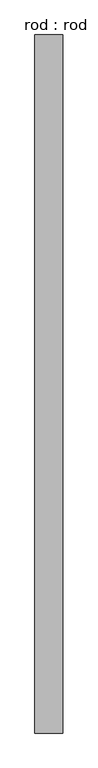
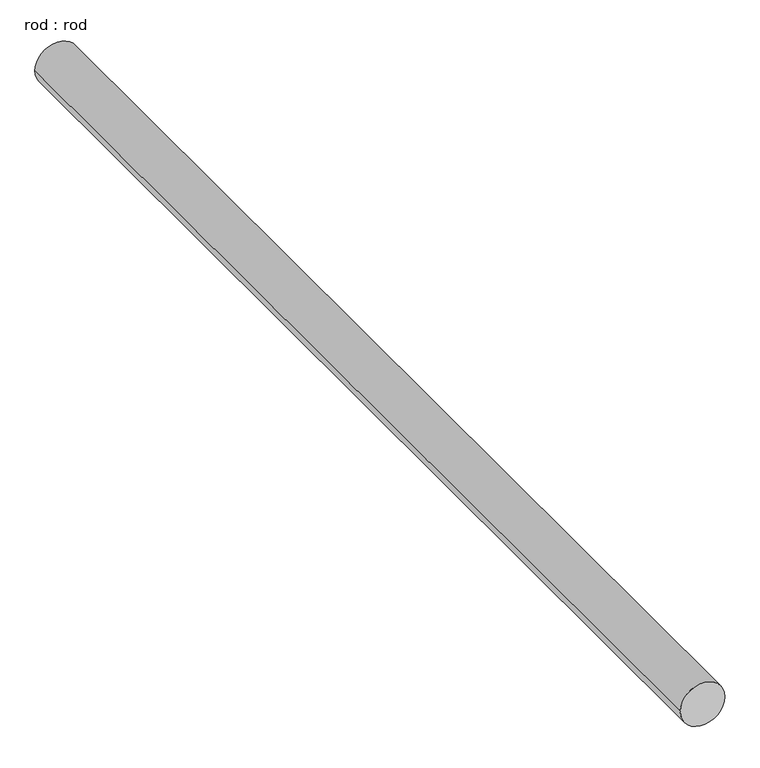
"""IFC4 building model written with IfcOpenShell, lengths in millimetres: proxy geometry, rod : rod."""

import ifcopenshell
import ifcopenshell.guid

model = None  # the IFC model being written
_history = None  # IfcOwnerHistory: only IFC2X3 demands one
_inside = {}  # id of a spatial element -> (the spatial element, [elements in it])
_under = {}  # id of a project, library or spatial element -> (it, [spatial elements below it])
_declared = {}  # id of a project -> (the project, [libraries it declares])
_typed = {}  # id of a type object -> (the type object, [elements of that type])
_made_of = {}  # id of a material, layer set ... -> (it, [elements and type objects made of it])


def new_model(schema):
    """Start an empty IFC model of exactly this schema.

    Asked for "IFC4X3", IfcOpenShell would pick the latest addendum, in which some entities
    have other attributes; the version numbers below select the first issue.
    IFC2X3 requires an IfcOwnerHistory on every rooted entity: one is made here for all.
    """
    global model, _history
    if schema == "IFC4X3":
        model = ifcopenshell.file(schema_version=(4, 3, 0, 0))
    else:
        model = ifcopenshell.file(schema=schema)
    _inside.clear()
    _under.clear()
    _declared.clear()
    _typed.clear()
    _made_of.clear()
    _history = None
    if model.schema == "IFC2X3":
        org = make("IfcOrganization", Name="unknown")
        user = make(
            "IfcPersonAndOrganization",
            ThePerson=make("IfcPerson", FamilyName="unknown"),
            TheOrganization=org,
        )
        app = make(
            "IfcApplication",
            ApplicationDeveloper=org,
            Version="unknown",
            ApplicationFullName="unknown",
            ApplicationIdentifier="unknown",
        )
        _history = make(
            "IfcOwnerHistory",
            OwningUser=user,
            OwningApplication=app,
            ChangeAction="ADDED",
            CreationDate=0,
        )
    return model


def make(cls, **values):
    """One entity of the class cls with the attributes given. An attribute that is None is left unset."""
    return model.create_entity(
        cls, **{name: value for name, value in values.items() if value is not None}
    )


def rooted(cls, **values):
    """An entity with a GlobalId (a new one), such as an element, a storey or a relation."""
    return make(cls, GlobalId=ifcopenshell.guid.new(), OwnerHistory=_history, **values)


def si_unit(unit_type, name, prefix=None):
    """IfcSIUnit, for example si_unit("LENGTHUNIT", "METRE", prefix="MILLI")."""
    return make("IfcSIUnit", UnitType=unit_type, Prefix=prefix, Name=name)


def assignment(units):
    """IfcUnitAssignment: the units of a project."""
    return None if units is None else make("IfcUnitAssignment", Units=units)


def point(xyz):
    """IfcCartesianPoint."""
    return None if xyz is None else make("IfcCartesianPoint", Coordinates=xyz)


def direction(xyz):
    """IfcDirection."""
    return None if xyz is None else make("IfcDirection", DirectionRatios=xyz)


def frame(location, z_axis=None, x_axis=None):
    """IfcAxis2Placement3D, a coordinate frame: its origin and axes. An axis left out is left unset."""
    return make(
        "IfcAxis2Placement3D",
        Location=point(location),
        Axis=direction(z_axis),
        RefDirection=direction(x_axis),
    )


def frame_2d(location, x_axis=None):
    """IfcAxis2Placement2D, a coordinate frame in the plane: its origin and x axis."""
    return make(
        "IfcAxis2Placement2D", Location=point(location), RefDirection=direction(x_axis)
    )


def origin():
    """The frame at (0, 0, 0) with its axes left unset."""
    return frame((0.0, 0.0, 0.0))


def place(relative_to, where):
    """IfcLocalPlacement: puts the frame where relative to a parent placement (None: the world)."""
    return make(
        "IfcLocalPlacement", PlacementRelTo=relative_to, RelativePlacement=where
    )


def context(
    kind, dimensions, precision=None, world=None, true_north=None, identifier=None
):
    """IfcGeometricRepresentationContext, for example the 3D "Model" context."""
    return make(
        "IfcGeometricRepresentationContext",
        ContextIdentifier=identifier,
        ContextType=kind,
        CoordinateSpaceDimension=dimensions,
        Precision=precision,
        WorldCoordinateSystem=world,
        TrueNorth=true_north,
    )


def project(units=None, contexts=None):
    """IfcProject with its units and contexts."""
    return rooted(
        "IfcProject",
        Name="project",
        RepresentationContexts=contexts,
        UnitsInContext=assignment(units),
    )


def spatial(cls, under=None, at=None, **own):
    """A site, building, storey or space (cls), placed at a placement, below another one or the project."""
    s = rooted(cls, ObjectPlacement=at, **own)
    if under is not None:
        _under.setdefault(under.id(), (under, []))[1].append(s)
    return s


def circle_curve(where, radius):
    """IfcCircle in the frame where."""
    return make("IfcCircle", Position=where, Radius=radius)


def trimmed(basis, trim1, trim2, sense, master):
    """IfcTrimmedCurve: the piece of a basis curve between two trims."""
    return make(
        "IfcTrimmedCurve",
        BasisCurve=basis,
        Trim1=trim1,
        Trim2=trim2,
        SenseAgreement=sense,
        MasterRepresentation=master,
    )


def segment(curve, same_sense, transition):
    """IfcCompositeCurveSegment."""
    return make(
        "IfcCompositeCurveSegment",
        Transition=transition,
        SameSense=same_sense,
        ParentCurve=curve,
    )


def composite_curve(segments, self_intersect=None):
    """IfcCompositeCurve: segments joined end to end."""
    return make("IfcCompositeCurve", Segments=segments, SelfIntersect=self_intersect)


def outline(outer, holes=None, kind="AREA"):
    """IfcArbitraryClosedProfileDef: a profile drawn as a closed curve; with holes, ...WithVoids."""
    if holes is None:
        return make("IfcArbitraryClosedProfileDef", ProfileType=kind, OuterCurve=outer)
    return make(
        "IfcArbitraryProfileDefWithVoids",
        ProfileType=kind,
        OuterCurve=outer,
        InnerCurves=holes,
    )


def extrude(swept, where, along, depth):
    """IfcExtrudedAreaSolid: the profile swept, set in the frame where, extruded along a direction by depth."""
    return make(
        "IfcExtrudedAreaSolid",
        SweptArea=swept,
        Position=where,
        ExtrudedDirection=direction(along),
        Depth=depth,
    )


def shape(context_of_items, identifier, shape_type, items):
    """IfcShapeRepresentation: the items that make up one representation, for example the "Body"."""
    return make(
        "IfcShapeRepresentation",
        ContextOfItems=context_of_items,
        RepresentationIdentifier=identifier,
        RepresentationType=shape_type,
        Items=items,
    )


def source(mapping_origin, context_of_items, identifier, shape_type, items):
    """IfcRepresentationMap: a shape defined once, which mapped items show again and again."""
    return make(
        "IfcRepresentationMap",
        MappingOrigin=mapping_origin,
        MappedRepresentation=shape(context_of_items, identifier, shape_type, items),
    )


def transform(
    local_origin,
    x_axis=None,
    y_axis=None,
    z_axis=None,
    scale=None,
    scale2=None,
    scale3=None,
    uniform=True,
):
    """IfcCartesianTransformationOperator3D, or its non-uniform kind. x_axis, y_axis, z_axis: its Axis1, 2, 3."""
    if uniform:
        return make(
            "IfcCartesianTransformationOperator3D",
            Axis1=direction(x_axis),
            Axis2=direction(y_axis),
            LocalOrigin=point(local_origin),
            Scale=scale,
            Axis3=direction(z_axis),
        )
    return make(
        "IfcCartesianTransformationOperator3DnonUniform",
        Axis1=direction(x_axis),
        Axis2=direction(y_axis),
        LocalOrigin=point(local_origin),
        Scale=scale,
        Axis3=direction(z_axis),
        Scale2=scale2,
        Scale3=scale3,
    )


def mapped(mapping_source, mapping_target):
    """IfcMappedItem: shows the shape of a source again, moved by a transform."""
    return make(
        "IfcMappedItem", MappingSource=mapping_source, MappingTarget=mapping_target
    )


def made_of(thing, what):
    """Note that an element or type object is made of a material, layer set ...; save() writes the relation."""
    if what is not None:
        _made_of.setdefault(what.id(), (what, []))[1].append(thing)
    return thing


def element(
    cls,
    number,
    at=None,
    inside=None,
    cuts=None,
    type_object=None,
    material=None,
    context=None,
    identifier="Body",
    shape_type=None,
    held_by="IfcProductDefinitionShape",
    body=None,
    shapes=None,
    **own,
):
    """One element of the class cls, such as IfcWall. Its Tag is "e" and its number.

    at: its placement. inside: the storey or other place that contains it. cuts: it is an
    opening in that element (IfcRelVoidsElement). A single representation is given by context,
    identifier, shape_type and body (its items); several are given by shapes. held_by: the class
    of the entity that holds the representations. save() writes the other relations.
    """
    e = rooted(cls, Tag="e%d" % number, ObjectPlacement=at, **own)
    if body is not None:
        shapes = [shape(context, identifier, shape_type, body)]
    if shapes is not None:
        e.Representation = make(held_by, Representations=shapes)
    if inside is not None:
        _inside.setdefault(inside.id(), (inside, []))[1].append(e)
    if cuts is not None:
        rooted(
            "IfcRelVoidsElement", RelatingBuildingElement=cuts, RelatedOpeningElement=e
        )
    if type_object is not None:
        _typed.setdefault(type_object.id(), (type_object, []))[1].append(e)
    return made_of(e, material)


def aggregate(whole, parts):
    """IfcRelAggregates: a whole, such as a stair, and the parts it consists of."""
    return rooted("IfcRelAggregates", RelatingObject=whole, RelatedObjects=parts)


def save(model, path):
    """Write the relations noted so far, then the file.

    IfcRelAggregates (storeys below a building ...), IfcRelContainedInSpatialStructure (elements
    in a storey), IfcRelDefinesByType, IfcRelAssociatesMaterial and IfcRelDeclares: one each for
    every whole, place, type object, material and project.
    """
    for whole, parts in _under.values():
        aggregate(whole, parts)
    for where, things in _inside.values():
        rooted(
            "IfcRelContainedInSpatialStructure",
            RelatedElements=things,
            RelatingStructure=where,
        )
    for kind, things in _typed.values():
        rooted("IfcRelDefinesByType", RelatedObjects=things, RelatingType=kind)
    for what, things in _made_of.values():
        rooted("IfcRelAssociatesMaterial", RelatedObjects=things, RelatingMaterial=what)
    for by, libraries in _declared.values():
        rooted("IfcRelDeclares", RelatingContext=by, RelatedDefinitions=libraries)
    model.write(path)


def rod_rod_b4eebbc3(model_context):
    return source(origin(), model_context, "Body", "SweptSolid", [
        extrude(outline(composite_curve([segment(trimmed(circle_curve(frame_2d((0.0108462, 0.0)), 200.0), [point((0.0108462, 200.0))], [point((0.0108462, -200.0))], False, "CARTESIAN"), True, "CONTINUOUS"), segment(trimmed(circle_curve(frame_2d((0.0108462, 0.0)), 200.0), [point((0.0108462, -200.0))], [point((0.0108462, 200.0))], False, "CARTESIAN"), True, "CONTINUOUS")], self_intersect=False)), frame((0.0, -907.2713847, 0.0), z_axis=(0.0, 1.0, 0.0), x_axis=(0.0, 0.0, 1.0)), (0.0, 0.0, 1.0), 10000.0),
    ])


if __name__ == "__main__":
    model = new_model("IFC4")
    model_context = context("Model", 3, world=origin())
    ifc_project = project(units=[si_unit("LENGTHUNIT", "METRE", prefix="MILLI")], contexts=[model_context])
    site = spatial("IfcSite", under=ifc_project)
    building = spatial("IfcBuilding", under=site)
    placement = place(None, origin())
    rod_rod_shape = rod_rod_b4eebbc3(model_context)
    element("IfcBuildingElementProxy", 1, Name="rod : rod", ObjectType="rod : rod", at=placement, inside=building, context=model_context, shape_type="MappedRepresentation", body=[
        mapped(rod_rod_shape, transform((0.0, 0.0, 0.0), x_axis=(1.0, 0.0, 0.0), y_axis=(0.0, 1.0, 0.0), z_axis=(0.0, 0.0, 1.0))),
    ])
    save(model, "model.ifc")

# Revit data of these elements
# Type "rod : rod"
#   Default Elevation = 0
